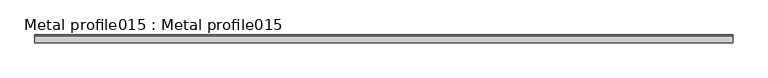
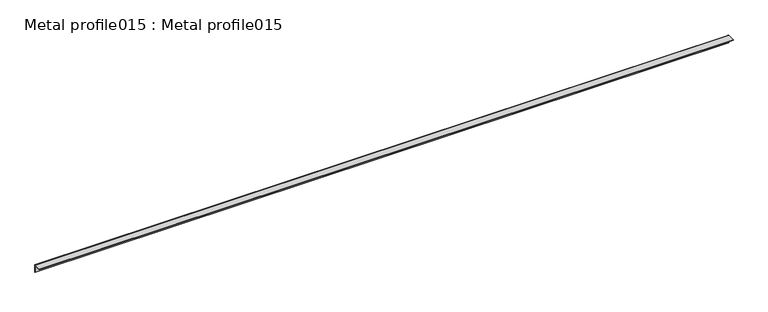
"""IFC4 building model written with IfcOpenShell, lengths in millimetres: proxy geometry, Metal profile015 : Metal profile015."""

import ifcopenshell
import ifcopenshell.guid

model = None  # the IFC model being written
_history = None  # IfcOwnerHistory: only IFC2X3 demands one
_inside = {}  # id of a spatial element -> (the spatial element, [elements in it])
_under = {}  # id of a project, library or spatial element -> (it, [spatial elements below it])
_declared = {}  # id of a project -> (the project, [libraries it declares])
_typed = {}  # id of a type object -> (the type object, [elements of that type])
_made_of = {}  # id of a material, layer set ... -> (it, [elements and type objects made of it])


def new_model(schema):
    """Start an empty IFC model of exactly this schema.

    Asked for "IFC4X3", IfcOpenShell would pick the latest addendum, in which some entities
    have other attributes; the version numbers below select the first issue.
    IFC2X3 requires an IfcOwnerHistory on every rooted entity: one is made here for all.
    """
    global model, _history
    if schema == "IFC4X3":
        model = ifcopenshell.file(schema_version=(4, 3, 0, 0))
    else:
        model = ifcopenshell.file(schema=schema)
    _inside.clear()
    _under.clear()
    _declared.clear()
    _typed.clear()
    _made_of.clear()
    _history = None
    if model.schema == "IFC2X3":
        org = make("IfcOrganization", Name="unknown")
        user = make(
            "IfcPersonAndOrganization",
            ThePerson=make("IfcPerson", FamilyName="unknown"),
            TheOrganization=org,
        )
        app = make(
            "IfcApplication",
            ApplicationDeveloper=org,
            Version="unknown",
            ApplicationFullName="unknown",
            ApplicationIdentifier="unknown",
        )
        _history = make(
            "IfcOwnerHistory",
            OwningUser=user,
            OwningApplication=app,
            ChangeAction="ADDED",
            CreationDate=0,
        )
    return model


def make(cls, **values):
    """One entity of the class cls with the attributes given. An attribute that is None is left unset."""
    return model.create_entity(
        cls, **{name: value for name, value in values.items() if value is not None}
    )


def rooted(cls, **values):
    """An entity with a GlobalId (a new one), such as an element, a storey or a relation."""
    return make(cls, GlobalId=ifcopenshell.guid.new(), OwnerHistory=_history, **values)


def si_unit(unit_type, name, prefix=None):
    """IfcSIUnit, for example si_unit("LENGTHUNIT", "METRE", prefix="MILLI")."""
    return make("IfcSIUnit", UnitType=unit_type, Prefix=prefix, Name=name)


def assignment(units):
    """IfcUnitAssignment: the units of a project."""
    return None if units is None else make("IfcUnitAssignment", Units=units)


def point(xyz):
    """IfcCartesianPoint."""
    return None if xyz is None else make("IfcCartesianPoint", Coordinates=xyz)


def direction(xyz):
    """IfcDirection."""
    return None if xyz is None else make("IfcDirection", DirectionRatios=xyz)


def frame(location, z_axis=None, x_axis=None):
    """IfcAxis2Placement3D, a coordinate frame: its origin and axes. An axis left out is left unset."""
    return make(
        "IfcAxis2Placement3D",
        Location=point(location),
        Axis=direction(z_axis),
        RefDirection=direction(x_axis),
    )


def frame_2d(location, x_axis=None):
    """IfcAxis2Placement2D, a coordinate frame in the plane: its origin and x axis."""
    return make(
        "IfcAxis2Placement2D", Location=point(location), RefDirection=direction(x_axis)
    )


def origin():
    """The frame at (0, 0, 0) with its axes left unset."""
    return frame((0.0, 0.0, 0.0))


def place(relative_to, where):
    """IfcLocalPlacement: puts the frame where relative to a parent placement (None: the world)."""
    return make(
        "IfcLocalPlacement", PlacementRelTo=relative_to, RelativePlacement=where
    )


def context(
    kind, dimensions, precision=None, world=None, true_north=None, identifier=None
):
    """IfcGeometricRepresentationContext, for example the 3D "Model" context."""
    return make(
        "IfcGeometricRepresentationContext",
        ContextIdentifier=identifier,
        ContextType=kind,
        CoordinateSpaceDimension=dimensions,
        Precision=precision,
        WorldCoordinateSystem=world,
        TrueNorth=true_north,
    )


def project(units=None, contexts=None):
    """IfcProject with its units and contexts."""
    return rooted(
        "IfcProject",
        Name="project",
        RepresentationContexts=contexts,
        UnitsInContext=assignment(units),
    )


def spatial(cls, under=None, at=None, **own):
    """A site, building, storey or space (cls), placed at a placement, below another one or the project."""
    s = rooted(cls, ObjectPlacement=at, **own)
    if under is not None:
        _under.setdefault(under.id(), (under, []))[1].append(s)
    return s


def polyline(points):
    """IfcPolyline through the points."""
    return make("IfcPolyline", Points=[point(p) for p in points])


def circle_curve(where, radius):
    """IfcCircle in the frame where."""
    return make("IfcCircle", Position=where, Radius=radius)


def trimmed(basis, trim1, trim2, sense, master):
    """IfcTrimmedCurve: the piece of a basis curve between two trims."""
    return make(
        "IfcTrimmedCurve",
        BasisCurve=basis,
        Trim1=trim1,
        Trim2=trim2,
        SenseAgreement=sense,
        MasterRepresentation=master,
    )


def segment(curve, same_sense, transition):
    """IfcCompositeCurveSegment."""
    return make(
        "IfcCompositeCurveSegment",
        Transition=transition,
        SameSense=same_sense,
        ParentCurve=curve,
    )


def composite_curve(segments, self_intersect=None):
    """IfcCompositeCurve: segments joined end to end."""
    return make("IfcCompositeCurve", Segments=segments, SelfIntersect=self_intersect)


def outline(outer, holes=None, kind="AREA"):
    """IfcArbitraryClosedProfileDef: a profile drawn as a closed curve; with holes, ...WithVoids."""
    if holes is None:
        return make("IfcArbitraryClosedProfileDef", ProfileType=kind, OuterCurve=outer)
    return make(
        "IfcArbitraryProfileDefWithVoids",
        ProfileType=kind,
        OuterCurve=outer,
        InnerCurves=holes,
    )


def extrude(swept, where, along, depth):
    """IfcExtrudedAreaSolid: the profile swept, set in the frame where, extruded along a direction by depth."""
    return make(
        "IfcExtrudedAreaSolid",
        SweptArea=swept,
        Position=where,
        ExtrudedDirection=direction(along),
        Depth=depth,
    )


def shape(context_of_items, identifier, shape_type, items):
    """IfcShapeRepresentation: the items that make up one representation, for example the "Body"."""
    return make(
        "IfcShapeRepresentation",
        ContextOfItems=context_of_items,
        RepresentationIdentifier=identifier,
        RepresentationType=shape_type,
        Items=items,
    )


def source(mapping_origin, context_of_items, identifier, shape_type, items):
    """IfcRepresentationMap: a shape defined once, which mapped items show again and again."""
    return make(
        "IfcRepresentationMap",
        MappingOrigin=mapping_origin,
        MappedRepresentation=shape(context_of_items, identifier, shape_type, items),
    )


def transform(
    local_origin,
    x_axis=None,
    y_axis=None,
    z_axis=None,
    scale=None,
    scale2=None,
    scale3=None,
    uniform=True,
):
    """IfcCartesianTransformationOperator3D, or its non-uniform kind. x_axis, y_axis, z_axis: its Axis1, 2, 3."""
    if uniform:
        return make(
            "IfcCartesianTransformationOperator3D",
            Axis1=direction(x_axis),
            Axis2=direction(y_axis),
            LocalOrigin=point(local_origin),
            Scale=scale,
            Axis3=direction(z_axis),
        )
    return make(
        "IfcCartesianTransformationOperator3DnonUniform",
        Axis1=direction(x_axis),
        Axis2=direction(y_axis),
        LocalOrigin=point(local_origin),
        Scale=scale,
        Axis3=direction(z_axis),
        Scale2=scale2,
        Scale3=scale3,
    )


def mapped(mapping_source, mapping_target):
    """IfcMappedItem: shows the shape of a source again, moved by a transform."""
    return make(
        "IfcMappedItem", MappingSource=mapping_source, MappingTarget=mapping_target
    )


def made_of(thing, what):
    """Note that an element or type object is made of a material, layer set ...; save() writes the relation."""
    if what is not None:
        _made_of.setdefault(what.id(), (what, []))[1].append(thing)
    return thing


def element(
    cls,
    number,
    at=None,
    inside=None,
    cuts=None,
    type_object=None,
    material=None,
    context=None,
    identifier="Body",
    shape_type=None,
    held_by="IfcProductDefinitionShape",
    body=None,
    shapes=None,
    **own,
):
    """One element of the class cls, such as IfcWall. Its Tag is "e" and its number.

    at: its placement. inside: the storey or other place that contains it. cuts: it is an
    opening in that element (IfcRelVoidsElement). A single representation is given by context,
    identifier, shape_type and body (its items); several are given by shapes. held_by: the class
    of the entity that holds the representations. save() writes the other relations.
    """
    e = rooted(cls, Tag="e%d" % number, ObjectPlacement=at, **own)
    if body is not None:
        shapes = [shape(context, identifier, shape_type, body)]
    if shapes is not None:
        e.Representation = make(held_by, Representations=shapes)
    if inside is not None:
        _inside.setdefault(inside.id(), (inside, []))[1].append(e)
    if cuts is not None:
        rooted(
            "IfcRelVoidsElement", RelatingBuildingElement=cuts, RelatedOpeningElement=e
        )
    if type_object is not None:
        _typed.setdefault(type_object.id(), (type_object, []))[1].append(e)
    return made_of(e, material)


def aggregate(whole, parts):
    """IfcRelAggregates: a whole, such as a stair, and the parts it consists of."""
    return rooted("IfcRelAggregates", RelatingObject=whole, RelatedObjects=parts)


def save(model, path):
    """Write the relations noted so far, then the file.

    IfcRelAggregates (storeys below a building ...), IfcRelContainedInSpatialStructure (elements
    in a storey), IfcRelDefinesByType, IfcRelAssociatesMaterial and IfcRelDeclares: one each for
    every whole, place, type object, material and project.
    """
    for whole, parts in _under.values():
        aggregate(whole, parts)
    for where, things in _inside.values():
        rooted(
            "IfcRelContainedInSpatialStructure",
            RelatedElements=things,
            RelatingStructure=where,
        )
    for kind, things in _typed.values():
        rooted("IfcRelDefinesByType", RelatedObjects=things, RelatingType=kind)
    for what, things in _made_of.values():
        rooted("IfcRelAssociatesMaterial", RelatedObjects=things, RelatingMaterial=what)
    for by, libraries in _declared.values():
        rooted("IfcRelDeclares", RelatingContext=by, RelatedDefinitions=libraries)
    model.write(path)


def metal_profile015_metal_profile015_1b71c693(model_context):
    return source(origin(), model_context, "Body", "SweptSolid", [
        extrude(outline(composite_curve([segment(polyline([(-4258.3374811, 41076.616), (-4258.3374811, 41077.896), (-4237.4345714, 41077.896)]), True, "CONTINUOUS"), segment(trimmed(circle_curve(frame_2d((-4236.5442972, 41077.256)), 1.0964434), [point((-4237.4345714, 41077.896))], [point((-4235.9042972, 41076.3657258))], False, "CARTESIAN"), True, "CONTINUOUS"), segment(polyline([(-4235.9042972, 41076.3657258), (-4235.9042972, 41055.4628161), (-4237.1842972, 41055.4628161), (-4237.1842972, 41076.616), (-4258.3374811, 41076.616)]), True, "CONTINUOUS")], self_intersect=False)), frame((12383.0178845, 0.0, 0.0), z_axis=(1.0, 0.0, 0.0), x_axis=(0.0, 1.0, 0.0)), (0.0, 0.0, 1.0), 2000.0),
    ])


if __name__ == "__main__":
    model = new_model("IFC4")
    model_context = context("Model", 3, world=origin())
    ifc_project = project(units=[si_unit("LENGTHUNIT", "METRE", prefix="MILLI")], contexts=[model_context])
    site = spatial("IfcSite", under=ifc_project)
    building = spatial("IfcBuilding", under=site)
    placement = place(None, origin())
    metal_profile015_metal_profile015_shape = metal_profile015_metal_profile015_1b71c693(model_context)
    element("IfcBuildingElementProxy", 1, Name="Metal profile015 : Metal profile015", ObjectType="Metal profile015 : Metal profile015", at=placement, inside=building, context=model_context, shape_type="MappedRepresentation", body=[
        mapped(metal_profile015_metal_profile015_shape, transform((0.0, 0.0, 0.0), x_axis=(1.0, 0.0, 0.0), y_axis=(0.0, 1.0, 0.0), z_axis=(0.0, 0.0, 1.0))),
    ])
    save(model, "model.ifc")

# Revit data of these elements
# Type "Metal profile015 : Metal profile015"
#   NameOverride = "Metal profile015"
# Element 1 (IfcBuildingElementProxy, "Metal profile015 : Metal profile015")
#   Materials on its faces: "CORNER BEAD"
# Materials
#   "CORNER BEAD": class "Unassigned", colour RGB 255 241 0, transparency 0
